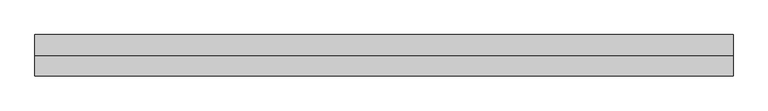
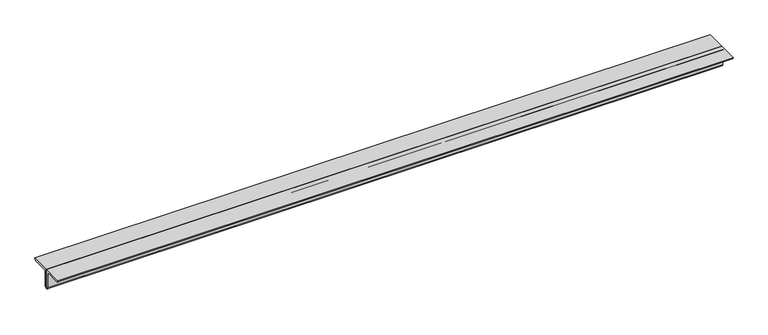
"""IFC4 building model written with IfcOpenShell, lengths in millimetres: member geometry, 0123_Steel Framing_2Ls-KSD3502 : H_SB_AR_S03_2Ls-130x130x12_HBR1."""

from ifc_helpers import new_model, si_unit, point, frame, frame_2d, origin, place, context, project, spatial, polyline, circle_curve, trimmed, segment, composite_curve, outline, extrude, source, transform, mapped, element, save


def member_50d2e036(model_context):
    return source(origin(), model_context, "Body", "SweptSolid", [
        extrude(outline(composite_curve([segment(polyline([(0.0, 36.4), (130.0, 36.4)]), True, "CONTINUOUS"), segment(trimmed(circle_curve(frame_2d((118.0, 36.4)), 12.0), [point((130.0, 36.4))], [point((118.0, 24.4))], False, "CARTESIAN"), True, "CONTINUOUS"), segment(polyline([(118.0, 24.4), (24.0, 24.4)]), True, "CONTINUOUS"), segment(trimmed(circle_curve(frame_2d((24.0, 12.4)), 12.0), [point((24.0, 24.4))], [point((12.0, 12.4))], True, "CARTESIAN"), True, "CONTINUOUS"), segment(polyline([(12.0, 12.4), (12.0, -81.6)]), True, "CONTINUOUS"), segment(trimmed(circle_curve(frame_2d((0.0, -81.6)), 12.0), [point((12.0, -81.6))], [point((0.0, -93.6))], False, "CARTESIAN"), True, "CONTINUOUS"), segment(polyline([(0.0, -93.6), (0.0, 36.4)]), True, "CONTINUOUS")], self_intersect=False)), frame((-2203.0201459, 0.0, 0.0), z_axis=(1.0, 0.0, 0.0), x_axis=(0.0, 1.0, 0.0)), (0.0, 0.0, 1.0), 4391.0649986),
        extrude(outline(composite_curve([segment(polyline([(0.0, 36.4), (0.0, -93.6)]), True, "CONTINUOUS"), segment(trimmed(circle_curve(frame_2d((0.0, -81.6)), 12.0), [point((0.0, -93.6))], [point((-12.0, -81.6))], False, "CARTESIAN"), True, "CONTINUOUS"), segment(polyline([(-12.0, -81.6), (-12.0, 12.4)]), True, "CONTINUOUS"), segment(trimmed(circle_curve(frame_2d((-24.0, 12.4)), 12.0), [point((-12.0, 12.4))], [point((-24.0, 24.4))], True, "CARTESIAN"), True, "CONTINUOUS"), segment(polyline([(-24.0, 24.4), (-118.0, 24.4)]), True, "CONTINUOUS"), segment(trimmed(circle_curve(frame_2d((-118.0, 36.4)), 12.0), [point((-118.0, 24.4))], [point((-130.0, 36.4))], False, "CARTESIAN"), True, "CONTINUOUS"), segment(polyline([(-130.0, 36.4), (0.0, 36.4)]), True, "CONTINUOUS")], self_intersect=False)), frame((-2203.0201459, 0.0, 0.0), z_axis=(1.0, 0.0, 0.0), x_axis=(0.0, 1.0, 0.0)), (0.0, 0.0, 1.0), 4391.0649986),
    ])


if __name__ == "__main__":
    model = new_model("IFC4")
    model_context = context("Model", 3, world=origin())
    ifc_project = project(units=[si_unit("LENGTHUNIT", "METRE", prefix="MILLI")], contexts=[model_context])
    site = spatial("IfcSite", under=ifc_project)
    building = spatial("IfcBuilding", under=site)
    placement = place(None, origin())
    member_shape = member_50d2e036(model_context)
    element("IfcMember", 1, ObjectType="0123_Steel Framing_2Ls-KSD3502 : H_SB_AR_S03_2Ls-130x130x12_HBR1", at=placement, inside=building, context=model_context, shape_type="MappedRepresentation", body=[
        mapped(member_shape, transform((0.0, 0.0, 0.0), x_axis=(1.0, 0.0, 0.0), y_axis=(0.0, 1.0, 0.0), z_axis=(0.0, 0.0, 1.0))),
    ])
    save(model, "model.ifc")

# Revit data of these elements
# Type "0123_Steel Framing_2Ls-KSD3502 : H_SB_AR_S03_2Ls-130x130x12_HBR1"
#   Assembly Code = "B10"
#   Legs = "SLBB"
#   W = 8.97
#   Perimeter = 1.04 m²/m
#   Nominal Weight = 46.80 kgf/m
#   Length [instance default] = 1000 mm
#   Space = 0 mm
#   b = 130 mm
#   d = 130 mm
#   t = 12 mm
#   y = 36.4 mm
#   A = 0.005952 m²
#   Structural Material [instance default] = Steel ASTM A36
# Element 1 (IfcMember, "0123_Steel Framing_2Ls-KSD3502 : H_SB_AR_S03_2Ls-130x130x12_HBR1")
#   Structural Material = Steel, 45-345
#   Materials on its faces: "Steel, 45-345"
# Materials
#   "Steel ASTM A36": class "Metal", colour RGB 199 199 199, transparency 0, Description = "Structural steel, ASTM A36 Grade B, mill finish", Cost = 0
#   "Steel, 45-345": class "Metal", colour RGB 189 187 185, transparency 0, Description = "Steel 345 MPa", Cost = 0
